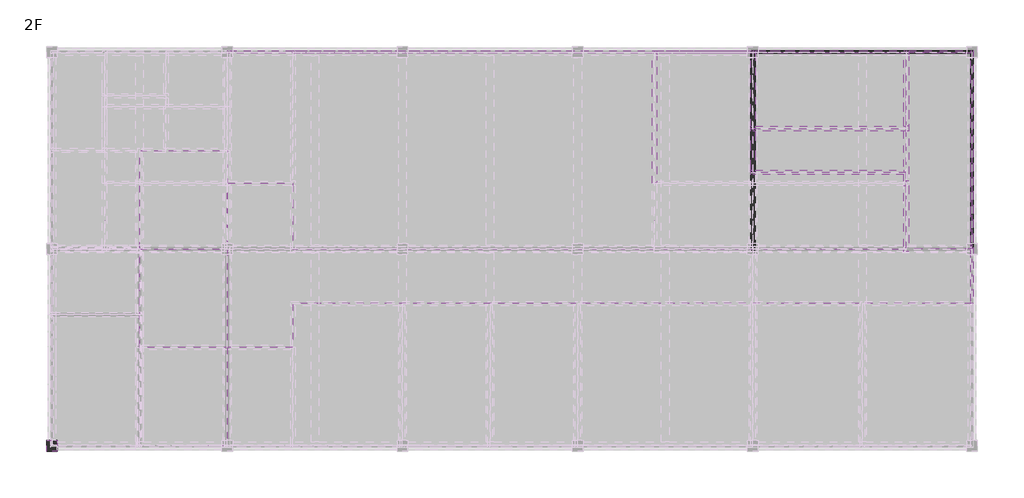
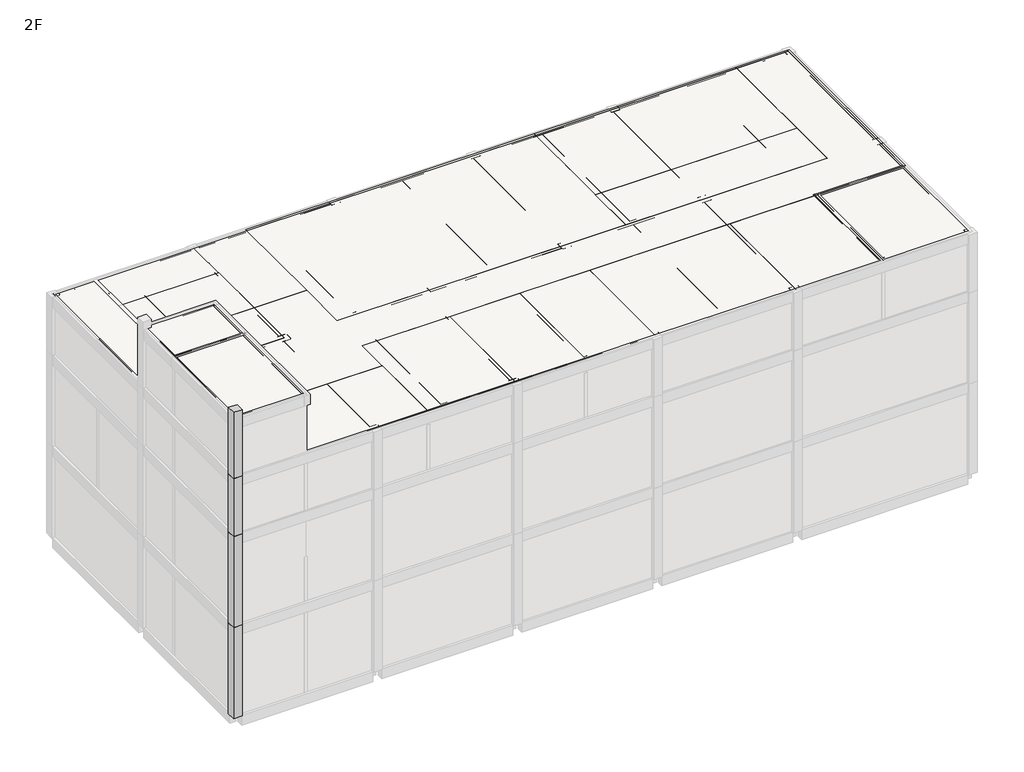
# One storey, part 3 of 7: 58 slabs, 19 walls, 4 columns.
"""IFC4 building model written with IfcOpenShell, lengths in millimetres."""

import ifcopenshell
import ifcopenshell.guid

model = None  # the IFC model being written
_history = None  # IfcOwnerHistory: only IFC2X3 demands one
_inside = {}  # id of a spatial element -> (the spatial element, [elements in it])
_under = {}  # id of a project, library or spatial element -> (it, [spatial elements below it])
_declared = {}  # id of a project -> (the project, [libraries it declares])
_typed = {}  # id of a type object -> (the type object, [elements of that type])
_made_of = {}  # id of a material, layer set ... -> (it, [elements and type objects made of it])


def new_model(schema):
    """Start an empty IFC model of exactly this schema.

    Asked for "IFC4X3", IfcOpenShell would pick the latest addendum, in which some entities
    have other attributes; the version numbers below select the first issue.
    IFC2X3 requires an IfcOwnerHistory on every rooted entity: one is made here for all.
    """
    global model, _history
    if schema == "IFC4X3":
        model = ifcopenshell.file(schema_version=(4, 3, 0, 0))
    else:
        model = ifcopenshell.file(schema=schema)
    _inside.clear()
    _under.clear()
    _declared.clear()
    _typed.clear()
    _made_of.clear()
    _history = None
    if model.schema == "IFC2X3":
        org = make("IfcOrganization", Name="unknown")
        user = make(
            "IfcPersonAndOrganization",
            ThePerson=make("IfcPerson", FamilyName="unknown"),
            TheOrganization=org,
        )
        app = make(
            "IfcApplication",
            ApplicationDeveloper=org,
            Version="unknown",
            ApplicationFullName="unknown",
            ApplicationIdentifier="unknown",
        )
        _history = make(
            "IfcOwnerHistory",
            OwningUser=user,
            OwningApplication=app,
            ChangeAction="ADDED",
            CreationDate=0,
        )
    return model


def make(cls, **values):
    """One entity of the class cls with the attributes given. An attribute that is None is left unset."""
    return model.create_entity(
        cls, **{name: value for name, value in values.items() if value is not None}
    )


def rooted(cls, **values):
    """An entity with a GlobalId (a new one), such as an element, a storey or a relation."""
    return make(cls, GlobalId=ifcopenshell.guid.new(), OwnerHistory=_history, **values)


def si_unit(unit_type, name, prefix=None):
    """IfcSIUnit, for example si_unit("LENGTHUNIT", "METRE", prefix="MILLI")."""
    return make("IfcSIUnit", UnitType=unit_type, Prefix=prefix, Name=name)


def assignment(units):
    """IfcUnitAssignment: the units of a project."""
    return None if units is None else make("IfcUnitAssignment", Units=units)


def point(xyz):
    """IfcCartesianPoint."""
    return None if xyz is None else make("IfcCartesianPoint", Coordinates=xyz)


def direction(xyz):
    """IfcDirection."""
    return None if xyz is None else make("IfcDirection", DirectionRatios=xyz)


def frame(location, z_axis=None, x_axis=None):
    """IfcAxis2Placement3D, a coordinate frame: its origin and axes. An axis left out is left unset."""
    return make(
        "IfcAxis2Placement3D",
        Location=point(location),
        Axis=direction(z_axis),
        RefDirection=direction(x_axis),
    )


def origin():
    """The frame at (0, 0, 0) with its axes left unset."""
    return frame((0.0, 0.0, 0.0))


def place(relative_to, where):
    """IfcLocalPlacement: puts the frame where relative to a parent placement (None: the world)."""
    return make(
        "IfcLocalPlacement", PlacementRelTo=relative_to, RelativePlacement=where
    )


def context(
    kind, dimensions, precision=None, world=None, true_north=None, identifier=None
):
    """IfcGeometricRepresentationContext, for example the 3D "Model" context."""
    return make(
        "IfcGeometricRepresentationContext",
        ContextIdentifier=identifier,
        ContextType=kind,
        CoordinateSpaceDimension=dimensions,
        Precision=precision,
        WorldCoordinateSystem=world,
        TrueNorth=true_north,
    )


def project(units=None, contexts=None):
    """IfcProject with its units and contexts."""
    return rooted(
        "IfcProject",
        Name="project",
        RepresentationContexts=contexts,
        UnitsInContext=assignment(units),
    )


def spatial(cls, under=None, at=None, **own):
    """A site, building, storey or space (cls), placed at a placement, below another one or the project."""
    s = rooted(cls, ObjectPlacement=at, **own)
    if under is not None:
        _under.setdefault(under.id(), (under, []))[1].append(s)
    return s


def polyline(points):
    """IfcPolyline through the points."""
    return make("IfcPolyline", Points=[point(p) for p in points])


def outline(outer, holes=None, kind="AREA"):
    """IfcArbitraryClosedProfileDef: a profile drawn as a closed curve; with holes, ...WithVoids."""
    if holes is None:
        return make("IfcArbitraryClosedProfileDef", ProfileType=kind, OuterCurve=outer)
    return make(
        "IfcArbitraryProfileDefWithVoids",
        ProfileType=kind,
        OuterCurve=outer,
        InnerCurves=holes,
    )


def extrude(swept, where, along, depth):
    """IfcExtrudedAreaSolid: the profile swept, set in the frame where, extruded along a direction by depth."""
    return make(
        "IfcExtrudedAreaSolid",
        SweptArea=swept,
        Position=where,
        ExtrudedDirection=direction(along),
        Depth=depth,
    )


def faces_of(points, faces, orient=None, outer=None):
    """IfcFace entities. A face is a list of loops; a loop is a list of indices into points, from 0.

    orient and outer hold one flag for each loop. By default every Orientation is true, the
    first loop of a face is its IfcFaceOuterBound and the others are IfcFaceBound.
    """
    made = []
    for i, loops in enumerate(faces):
        bounds = []
        for j, loop in enumerate(loops):
            is_outer = j == 0 if outer is None else outer[i][j]
            bounds.append(
                make(
                    "IfcFaceOuterBound" if is_outer else "IfcFaceBound",
                    Bound=make("IfcPolyLoop", Polygon=[points[k] for k in loop]),
                    Orientation=True if orient is None else orient[i][j],
                )
            )
        made.append(make("IfcFace", Bounds=bounds))
    return made


def faceted_brep(points, faces, orient=None, outer=None, voids=None):
    """IfcFacetedBrep: a solid bounded by flat faces; with voids (closed shells), ...WithVoids."""
    shared = [point(p) for p in points]
    hull = make("IfcClosedShell", CfsFaces=faces_of(shared, faces, orient, outer))
    if voids is None:
        return make("IfcFacetedBrep", Outer=hull)
    return make(
        "IfcFacetedBrepWithVoids",
        Outer=hull,
        Voids=[
            make(cls, CfsFaces=faces_of(shared, fs, o, b)) for cls, fs, o, b in voids
        ],
    )


def shape(context_of_items, identifier, shape_type, items):
    """IfcShapeRepresentation: the items that make up one representation, for example the "Body"."""
    return make(
        "IfcShapeRepresentation",
        ContextOfItems=context_of_items,
        RepresentationIdentifier=identifier,
        RepresentationType=shape_type,
        Items=items,
    )


def made_of(thing, what):
    """Note that an element or type object is made of a material, layer set ...; save() writes the relation."""
    if what is not None:
        _made_of.setdefault(what.id(), (what, []))[1].append(thing)
    return thing


def element(
    cls,
    number,
    at=None,
    inside=None,
    cuts=None,
    type_object=None,
    material=None,
    context=None,
    identifier="Body",
    shape_type=None,
    held_by="IfcProductDefinitionShape",
    body=None,
    shapes=None,
    **own,
):
    """One element of the class cls, such as IfcWall. Its Tag is "e" and its number.

    at: its placement. inside: the storey or other place that contains it. cuts: it is an
    opening in that element (IfcRelVoidsElement). A single representation is given by context,
    identifier, shape_type and body (its items); several are given by shapes. held_by: the class
    of the entity that holds the representations. save() writes the other relations.
    """
    e = rooted(cls, Tag="e%d" % number, ObjectPlacement=at, **own)
    if body is not None:
        shapes = [shape(context, identifier, shape_type, body)]
    if shapes is not None:
        e.Representation = make(held_by, Representations=shapes)
    if inside is not None:
        _inside.setdefault(inside.id(), (inside, []))[1].append(e)
    if cuts is not None:
        rooted(
            "IfcRelVoidsElement", RelatingBuildingElement=cuts, RelatedOpeningElement=e
        )
    if type_object is not None:
        _typed.setdefault(type_object.id(), (type_object, []))[1].append(e)
    return made_of(e, material)


def aggregate(whole, parts):
    """IfcRelAggregates: a whole, such as a stair, and the parts it consists of."""
    return rooted("IfcRelAggregates", RelatingObject=whole, RelatedObjects=parts)


def save(model, path):
    """Write the relations noted so far, then the file.

    IfcRelAggregates (storeys below a building ...), IfcRelContainedInSpatialStructure (elements
    in a storey), IfcRelDefinesByType, IfcRelAssociatesMaterial and IfcRelDeclares: one each for
    every whole, place, type object, material and project.
    """
    for whole, parts in _under.values():
        aggregate(whole, parts)
    for where, things in _inside.values():
        rooted(
            "IfcRelContainedInSpatialStructure",
            RelatedElements=things,
            RelatingStructure=where,
        )
    for kind, things in _typed.values():
        rooted("IfcRelDefinesByType", RelatedObjects=things, RelatingType=kind)
    for what, things in _made_of.values():
        rooted("IfcRelAssociatesMaterial", RelatedObjects=things, RelatingMaterial=what)
    for by, libraries in _declared.values():
        rooted("IfcRelDeclares", RelatingContext=by, RelatedDefinitions=libraries)
    model.write(path)


model = new_model("IFC4")

# Units and contexts
model_context = context("Model", 3, world=origin())
ifc_project = project(units=[si_unit("LENGTHUNIT", "METRE", prefix="MILLI")], contexts=[model_context])

# Site, building, storey
site = spatial("IfcSite", under=ifc_project)
building = spatial("IfcBuilding", under=site)
storey = spatial("IfcBuildingStorey", under=building, Name="2F", Elevation=3500.0)

# Columns
placement = place(None, origin())
element("IfcColumn", 1, ObjectType="Concrete-Rectangular-Column : CL111_500x500", at=placement, inside=storey, context=model_context, shape_type="SweptSolid", body=[
    extrude(outline(polyline([(45709.6521483, 164173.8614395), (45709.6521483, 163673.8614395), (45209.6521483, 163673.8614395), (45209.6521483, 164173.8614395), (45709.6521483, 164173.8614395)])), frame((0.0, 0.0, 18000.0), z_axis=(0.0, 0.0, 1.0), x_axis=(1.0, 0.0, 0.0)), (0.0, 0.0, 1.0), 4000.0),
])
element("IfcColumn", 2, ObjectType="Concrete-Rectangular-Column : CL111_500x500", at=placement, inside=storey, context=model_context, shape_type="Brep", body=[
    faceted_brep([(45709.6521483, 164173.8614395, 3500.0), (45709.6521483, 163673.8614395, 3500.0), (45209.6521483, 163673.8614395, 3500.0), (45209.6521483, 164173.8614395, 3500.0), (45709.6521483, 164173.8614395, 9000.0), (45709.6521483, 164098.8614395, 9000.0), (45709.6521483, 163748.8614395, 9000.0), (45709.6521483, 163673.8614395, 9000.0), (45209.6521483, 163673.8614395, 9000.0), (45209.6521483, 164173.8614395, 9000.0), (45284.6521483, 164173.8614395, 9000.0), (45634.6521483, 164173.8614395, 9000.0)], [[[0, 1, 2, 3]], [[4, 5, 6, 7, 1, 0]], [[7, 8, 2, 1]], [[8, 9, 3, 2]], [[9, 10, 11, 4, 0, 3]], [[4, 11, 10, 9, 8, 7, 6, 5]]]),
])
element("IfcColumn", 3, ObjectType="Concrete-Rectangular-Column : CL111_500x500", at=placement, inside=storey, context=model_context, shape_type="Brep", body=[
    faceted_brep([(45709.6521483, 164173.8614395, 9000.0), (45709.6521483, 163673.8614395, 9000.0), (45209.6521483, 163673.8614395, 9000.0), (45209.6521483, 164173.8614395, 9000.0), (45709.6521483, 164173.8614395, 14500.0), (45709.6521483, 164098.8614395, 14500.0), (45709.6521483, 163748.8614395, 14500.0), (45709.6521483, 163673.8614395, 14500.0), (45209.6521483, 163673.8614395, 14500.0), (45209.6521483, 164173.8614395, 14500.0), (45284.6521483, 164173.8614395, 14500.0), (45634.6521483, 164173.8614395, 14500.0)], [[[0, 1, 2, 3]], [[4, 5, 6, 7, 1, 0]], [[7, 8, 2, 1]], [[8, 9, 3, 2]], [[9, 10, 11, 4, 0, 3]], [[4, 11, 10, 9, 8, 7, 6, 5]]]),
])
element("IfcColumn", 4, ObjectType="Concrete-Rectangular-Column : CL111_500x500", at=placement, inside=storey, context=model_context, shape_type="Brep", body=[
    faceted_brep([(45709.6521483, 164173.8614395, 14500.0), (45709.6521483, 163673.8614395, 14500.0), (45209.6521483, 163673.8614395, 14500.0), (45209.6521483, 164173.8614395, 14500.0), (45709.6521483, 164173.8614395, 18000.0), (45709.6521483, 164098.8614395, 18000.0), (45709.6521483, 163748.8614395, 18000.0), (45709.6521483, 163673.8614395, 18000.0), (45209.6521483, 163673.8614395, 18000.0), (45209.6521483, 164173.8614395, 18000.0), (45284.6521483, 164173.8614395, 18000.0), (45634.6521483, 164173.8614395, 18000.0)], [[[0, 1, 2, 3]], [[4, 5, 6, 7, 1, 0]], [[7, 8, 2, 1]], [[8, 9, 3, 2]], [[9, 10, 11, 4, 0, 3]], [[4, 11, 10, 9, 8, 7, 6, 5]]]),
])

# Slabs
element("IfcSlab", 5, ObjectType="CFS11_Slab RC_T150", at=placement, inside=storey, context=model_context, shape_type="SweptSolid", body=[
    extrude(outline(polyline([(77459.6521483, 181923.8614395), (77459.6521483, 172923.8614395), (45459.6521483, 172923.8614395), (45459.6521483, 181923.8614395), (77459.6521483, 181923.8614395)])), frame((0.0, 0.0, 3350.0), z_axis=(0.0, 0.0, 1.0), x_axis=(1.0, 0.0, 0.0)), (0.0, 0.0, 1.0), 150.0),
])
element("IfcSlab", 6, ObjectType="CFS11_Slab RC_T150", at=placement, inside=storey, context=model_context, shape_type="SweptSolid", body=[
    extrude(outline(polyline([(53459.6521483, 163923.8614395), (53459.6521483, 172923.8614395), (87459.6521483, 172923.8614395), (87459.6521483, 163923.8614395), (53459.6521483, 163923.8614395)])), frame((0.0, 0.0, 3350.0), z_axis=(0.0, 0.0, 1.0), x_axis=(1.0, 0.0, 0.0)), (0.0, 0.0, 1.0), 150.0),
])
element("IfcSlab", 7, ObjectType="CFS11_Slab RC_T150", at=placement, inside=storey, context=model_context, shape_type="SweptSolid", body=[
    extrude(outline(polyline([(77459.6521483, 181923.8614395), (87459.6521483, 181923.8614395), (87459.6521483, 172923.8614395), (77459.6521483, 172923.8614395), (77459.6521483, 181923.8614395)])), frame((0.0, 0.0, 3350.0), z_axis=(0.0, 0.0, 1.0), x_axis=(1.0, 0.0, 0.0)), (0.0, 0.0, 1.0), 150.0),
])
element("IfcSlab", 8, ObjectType="CFS11_Slab RC_T150", at=placement, inside=storey, context=model_context, shape_type="SweptSolid", body=[
    extrude(outline(polyline([(53459.6521483, 172923.8614395), (53459.6521483, 163923.8614395), (49459.6521483, 163923.8614395), (49459.6521483, 172923.8614395), (53459.6521483, 172923.8614395)])), frame((0.0, 0.0, 3350.0), z_axis=(0.0, 0.0, 1.0), x_axis=(1.0, 0.0, 0.0)), (0.0, 0.0, 1.0), 150.0),
])
element("IfcSlab", 9, ObjectType="CFS11_Slab RC_T150", at=placement, inside=storey, context=model_context, shape_type="SweptSolid", body=[
    extrude(outline(polyline([(49459.6521483, 172923.8614395), (49459.6521483, 169923.8614395), (45459.6521483, 169923.8614395), (45459.6521483, 172923.8614395), (49459.6521483, 172923.8614395)])), frame((0.0, 0.0, 3350.0), z_axis=(0.0, 0.0, 1.0), x_axis=(1.0, 0.0, 0.0)), (0.0, 0.0, 1.0), 150.0),
])
element("IfcSlab", 10, ObjectType="CFS11_Slab RC_T150", at=placement, inside=storey, context=model_context, shape_type="SweptSolid", body=[
    extrude(outline(polyline([(49459.6521483, 163923.8614395), (45459.6521483, 163923.8614395), (45459.6521483, 169923.8614395), (49459.6521483, 169923.8614395), (49459.6521483, 163923.8614395)])), frame((0.0, 0.0, 3350.0), z_axis=(0.0, 0.0, 1.0), x_axis=(1.0, 0.0, 0.0)), (0.0, 0.0, 1.0), 150.0),
])
element("IfcSlab", 11, ObjectType="CFS11_Slab RC_T150", at=placement, inside=storey, context=model_context, shape_type="SweptSolid", body=[
    extrude(outline(polyline([(53459.6521483, 181923.8614395), (77459.6521483, 181923.8614395), (77459.6521483, 172923.8614395), (53459.6521483, 172923.8614395), (53459.6521483, 181923.8614395)])), frame((0.0, 0.0, 8850.0), z_axis=(0.0, 0.0, 1.0), x_axis=(1.0, 0.0, 0.0)), (0.0, 0.0, 1.0), 150.0),
])
element("IfcSlab", 12, ObjectType="CFS11_Slab RC_T150", at=placement, inside=storey, context=model_context, shape_type="SweptSolid", body=[
    extrude(outline(polyline([(77459.6521483, 172923.8614395), (77459.6521483, 163923.8614395), (53459.6521483, 163923.8614395), (53459.6521483, 172923.8614395), (77459.6521483, 172923.8614395)])), frame((0.0, 0.0, 8850.0), z_axis=(0.0, 0.0, 1.0), x_axis=(1.0, 0.0, 0.0)), (0.0, 0.0, 1.0), 150.0),
])
element("IfcSlab", 13, ObjectType="CFS11_Slab RC_T150", at=placement, inside=storey, context=model_context, shape_type="SweptSolid", body=[
    extrude(outline(polyline([(77459.6521483, 181923.8614395), (84459.6521483, 181923.8614395), (84459.6521483, 178423.8614395), (77459.6521483, 178423.8614395), (77459.6521483, 181923.8614395)])), frame((0.0, 0.0, 8850.0), z_axis=(0.0, 0.0, 1.0), x_axis=(1.0, 0.0, 0.0)), (0.0, 0.0, 1.0), 150.0),
])
element("IfcSlab", 14, ObjectType="CFS11_Slab RC_T150", at=placement, inside=storey, context=model_context, shape_type="SweptSolid", body=[
    extrude(outline(polyline([(77459.6521483, 163923.8614395), (77459.6521483, 172923.8614395), (87459.6521483, 172923.8614395), (87459.6521483, 163923.8614395), (77459.6521483, 163923.8614395)])), frame((0.0, 0.0, 8850.0), z_axis=(0.0, 0.0, 1.0), x_axis=(1.0, 0.0, 0.0)), (0.0, 0.0, 1.0), 150.0),
])
element("IfcSlab", 15, ObjectType="CFS11_Slab RC_T150", at=placement, inside=storey, context=model_context, shape_type="SweptSolid", body=[
    extrude(outline(polyline([(77459.6521483, 176423.8614395), (84459.6521483, 176423.8614395), (84459.6521483, 172923.8614395), (77459.6521483, 172923.8614395), (77459.6521483, 176423.8614395)])), frame((0.0, 0.0, 8850.0), z_axis=(0.0, 0.0, 1.0), x_axis=(1.0, 0.0, 0.0)), (0.0, 0.0, 1.0), 150.0),
])
element("IfcSlab", 16, ObjectType="CFS11_Slab RC_T150", at=placement, inside=storey, context=model_context, shape_type="SweptSolid", body=[
    extrude(outline(polyline([(45459.6521483, 181923.8614395), (47859.6521483, 181923.8614395), (47859.6521483, 177423.8614395), (45459.6521483, 177423.8614395), (45459.6521483, 181923.8614395)])), frame((0.0, 0.0, 8850.0), z_axis=(0.0, 0.0, 1.0), x_axis=(1.0, 0.0, 0.0)), (0.0, 0.0, 1.0), 150.0),
])
element("IfcSlab", 17, ObjectType="CFS11_Slab RC_T150", at=placement, inside=storey, context=model_context, shape_type="SweptSolid", body=[
    extrude(outline(polyline([(45459.6521483, 172923.8614395), (45459.6521483, 177423.8614395), (49459.6521483, 177423.8614395), (49459.6521483, 172923.8614395), (45459.6521483, 172923.8614395)])), frame((0.0, 0.0, 8850.0), z_axis=(0.0, 0.0, 1.0), x_axis=(1.0, 0.0, 0.0)), (0.0, 0.0, 1.0), 150.0),
])
element("IfcSlab", 18, ObjectType="CFS11_Slab RC_T150", at=placement, inside=storey, context=model_context, shape_type="SweptSolid", body=[
    extrude(outline(polyline([(53459.6521483, 177423.8614395), (50659.6521483, 177423.8614395), (50659.6521483, 181923.8614395), (53459.6521483, 181923.8614395), (53459.6521483, 177423.8614395)])), frame((0.0, 0.0, 8850.0), z_axis=(0.0, 0.0, 1.0), x_axis=(1.0, 0.0, 0.0)), (0.0, 0.0, 1.0), 150.0),
])
element("IfcSlab", 19, ObjectType="CFS11_Slab RC_T150", at=placement, inside=storey, context=model_context, shape_type="SweptSolid", body=[
    extrude(outline(polyline([(47859.6521483, 181923.8614395), (50659.6521483, 181923.8614395), (50659.6521483, 179923.8614395), (47859.6521483, 179923.8614395), (47859.6521483, 181923.8614395)])), frame((0.0, 0.0, 8850.0), z_axis=(0.0, 0.0, 1.0), x_axis=(1.0, 0.0, 0.0)), (0.0, 0.0, 1.0), 150.0),
])
element("IfcSlab", 20, ObjectType="CFS11_Slab RC_T150", at=placement, inside=storey, context=model_context, shape_type="SweptSolid", body=[
    extrude(outline(polyline([(47859.6521483, 179923.8614395), (50659.6521483, 179923.8614395), (50659.6521483, 177423.8614395), (47859.6521483, 177423.8614395), (47859.6521483, 179923.8614395)])), frame((0.0, 0.0, 8850.0), z_axis=(0.0, 0.0, 1.0), x_axis=(1.0, 0.0, 0.0)), (0.0, 0.0, 1.0), 150.0),
])
element("IfcSlab", 21, ObjectType="CFS11_Slab RC_T150", at=placement, inside=storey, context=model_context, shape_type="SweptSolid", body=[
    extrude(outline(polyline([(49459.6521483, 172923.8614395), (49459.6521483, 169923.8614395), (45459.6521483, 169923.8614395), (45459.6521483, 172923.8614395), (49459.6521483, 172923.8614395)])), frame((0.0, 0.0, 8850.0), z_axis=(0.0, 0.0, 1.0), x_axis=(1.0, 0.0, 0.0)), (0.0, 0.0, 1.0), 150.0),
])
element("IfcSlab", 22, ObjectType="CFS11_Slab RC_T150", at=placement, inside=storey, context=model_context, shape_type="SweptSolid", body=[
    extrude(outline(polyline([(49459.6521483, 169923.8614395), (49459.6521483, 163923.8614395), (45459.6521483, 163923.8614395), (45459.6521483, 169923.8614395), (49459.6521483, 169923.8614395)])), frame((0.0, 0.0, 8850.0), z_axis=(0.0, 0.0, 1.0), x_axis=(1.0, 0.0, 0.0)), (0.0, 0.0, 1.0), 150.0),
])
element("IfcSlab", 23, ObjectType="CFS11_Slab RC_T150", at=placement, inside=storey, context=model_context, shape_type="SweptSolid", body=[
    extrude(outline(polyline([(77459.6521483, 178423.8614395), (84459.6521483, 178423.8614395), (84459.6521483, 181923.8614395), (87459.6521483, 181923.8614395), (87459.6521483, 172923.8614395), (84459.6521483, 172923.8614395), (84459.6521483, 176423.8614395), (77459.6521483, 176423.8614395), (77459.6521483, 178423.8614395)])), frame((0.0, 0.0, 8850.0), z_axis=(0.0, 0.0, 1.0), x_axis=(1.0, 0.0, 0.0)), (0.0, 0.0, 1.0), 150.0),
])
element("IfcSlab", 24, ObjectType="CFS11_Slab RC_T150", at=placement, inside=storey, context=model_context, shape_type="SweptSolid", body=[
    extrude(outline(polyline([(49459.6521483, 177423.8614395), (53459.6521483, 177423.8614395), (53459.6521483, 163923.8614395), (49459.6521483, 163923.8614395), (49459.6521483, 177423.8614395)])), frame((0.0, 0.0, 8850.0), z_axis=(0.0, 0.0, 1.0), x_axis=(1.0, 0.0, 0.0)), (0.0, 0.0, 1.0), 150.0),
])
element("IfcSlab", 25, ObjectType="CFS11_Slab RC_T150", at=placement, inside=storey, context=model_context, shape_type="SweptSolid", body=[
    extrude(outline(polyline([(61459.6521483, 163923.8614395), (61459.6521483, 170423.8614395), (65459.6521483, 170423.8614395), (65459.6521483, 163923.8614395), (61459.6521483, 163923.8614395)])), frame((0.0, 0.0, 14350.0), z_axis=(0.0, 0.0, 1.0), x_axis=(1.0, 0.0, 0.0)), (0.0, 0.0, 1.0), 150.0),
])
element("IfcSlab", 26, ObjectType="CFS11_Slab RC_T150", at=placement, inside=storey, context=model_context, shape_type="SweptSolid", body=[
    extrude(outline(polyline([(65459.6521483, 170423.8614395), (69459.6521483, 170423.8614395), (69459.6521483, 163923.8614395), (65459.6521483, 163923.8614395), (65459.6521483, 170423.8614395)])), frame((0.0, 0.0, 14350.0), z_axis=(0.0, 0.0, 1.0), x_axis=(1.0, 0.0, 0.0)), (0.0, 0.0, 1.0), 150.0),
])
element("IfcSlab", 27, ObjectType="CFS11_Slab RC_T150", at=placement, inside=storey, context=model_context, shape_type="SweptSolid", body=[
    extrude(outline(polyline([(84459.6521483, 181923.8614395), (84459.6521483, 175923.8614395), (72959.6521483, 175923.8614395), (72959.6521483, 181923.8614395), (84459.6521483, 181923.8614395)])), frame((0.0, 0.0, 14350.0), z_axis=(0.0, 0.0, 1.0), x_axis=(1.0, 0.0, 0.0)), (0.0, 0.0, 1.0), 150.0),
])
element("IfcSlab", 28, ObjectType="CFS11_Slab RC_T150", at=placement, inside=storey, context=model_context, shape_type="SweptSolid", body=[
    extrude(outline(polyline([(69459.6521483, 170423.8614395), (77459.6521483, 170423.8614395), (77459.6521483, 163923.8614395), (69459.6521483, 163923.8614395), (69459.6521483, 170423.8614395)])), frame((0.0, 0.0, 14350.0), z_axis=(0.0, 0.0, 1.0), x_axis=(1.0, 0.0, 0.0)), (0.0, 0.0, 1.0), 150.0),
])
element("IfcSlab", 29, ObjectType="CFS11_Slab RC_T150", at=placement, inside=storey, context=model_context, shape_type="SweptSolid", body=[
    extrude(outline(polyline([(56459.6521483, 181923.8614395), (72959.6521483, 181923.8614395), (72959.6521483, 172923.8614395), (56459.6521483, 172923.8614395), (56459.6521483, 181923.8614395)])), frame((0.0, 0.0, 14350.0), z_axis=(0.0, 0.0, 1.0), x_axis=(1.0, 0.0, 0.0)), (0.0, 0.0, 1.0), 150.0),
])
element("IfcSlab", 30, ObjectType="CFS11_Slab RC_T150", at=placement, inside=storey, context=model_context, shape_type="SweptSolid", body=[
    extrude(outline(polyline([(77459.6521483, 170423.8614395), (82459.6521483, 170423.8614395), (82459.6521483, 163923.8614395), (77459.6521483, 163923.8614395), (77459.6521483, 170423.8614395)])), frame((0.0, 0.0, 14350.0), z_axis=(0.0, 0.0, 1.0), x_axis=(1.0, 0.0, 0.0)), (0.0, 0.0, 1.0), 150.0),
])
element("IfcSlab", 31, ObjectType="CFS11_Slab RC_T150", at=placement, inside=storey, context=model_context, shape_type="SweptSolid", body=[
    extrude(outline(polyline([(82459.6521483, 170423.8614395), (87459.6521483, 170423.8614395), (87459.6521483, 163923.8614395), (82459.6521483, 163923.8614395), (82459.6521483, 170423.8614395)])), frame((0.0, 0.0, 14350.0), z_axis=(0.0, 0.0, 1.0), x_axis=(1.0, 0.0, 0.0)), (0.0, 0.0, 1.0), 150.0),
])
element("IfcSlab", 32, ObjectType="CFS11_Slab RC_T150", at=placement, inside=storey, context=model_context, shape_type="SweptSolid", body=[
    extrude(outline(polyline([(84459.6521483, 175923.8614395), (84459.6521483, 172923.8614395), (72959.6521483, 172923.8614395), (72959.6521483, 175923.8614395), (84459.6521483, 175923.8614395)])), frame((0.0, 0.0, 14350.0), z_axis=(0.0, 0.0, 1.0), x_axis=(1.0, 0.0, 0.0)), (0.0, 0.0, 1.0), 150.0),
])
element("IfcSlab", 33, ObjectType="CFS11_Slab RC_T150", at=placement, inside=storey, context=model_context, shape_type="SweptSolid", body=[
    extrude(outline(polyline([(61459.6521483, 163923.8614395), (56459.6521483, 163923.8614395), (56459.6521483, 170423.8614395), (61459.6521483, 170423.8614395), (61459.6521483, 163923.8614395)])), frame((0.0, 0.0, 14350.0), z_axis=(0.0, 0.0, 1.0), x_axis=(1.0, 0.0, 0.0)), (0.0, 0.0, 1.0), 150.0),
])
element("IfcSlab", 34, ObjectType="CFS11_Slab RC_T150", at=placement, inside=storey, context=model_context, shape_type="SweptSolid", body=[
    extrude(outline(polyline([(56459.6521483, 163923.8614395), (49459.6521483, 163923.8614395), (49459.6521483, 168423.8614395), (56459.6521483, 168423.8614395), (56459.6521483, 163923.8614395)])), frame((0.0, 0.0, 14350.0), z_axis=(0.0, 0.0, 1.0), x_axis=(1.0, 0.0, 0.0)), (0.0, 0.0, 1.0), 150.0),
])
element("IfcSlab", 35, ObjectType="CFS11_Slab RC_T150", at=placement, inside=storey, context=model_context, shape_type="SweptSolid", body=[
    extrude(outline(polyline([(53459.6521483, 179423.8614395), (53459.6521483, 175923.8614395), (47859.6521483, 175923.8614395), (47859.6521483, 179423.8614395), (53459.6521483, 179423.8614395)])), frame((0.0, 0.0, 14350.0), z_axis=(0.0, 0.0, 1.0), x_axis=(1.0, 0.0, 0.0)), (0.0, 0.0, 1.0), 150.0),
])
element("IfcSlab", 36, ObjectType="CFS11_Slab RC_T150", at=placement, inside=storey, context=model_context, shape_type="SweptSolid", body=[
    extrude(outline(polyline([(47859.6521483, 179423.8614395), (47859.6521483, 181923.8614395), (53459.6521483, 181923.8614395), (53459.6521483, 179423.8614395), (47859.6521483, 179423.8614395)])), frame((0.0, 0.0, 14350.0), z_axis=(0.0, 0.0, 1.0), x_axis=(1.0, 0.0, 0.0)), (0.0, 0.0, 1.0), 150.0),
])
element("IfcSlab", 37, ObjectType="CFS11_Slab RC_T150", at=placement, inside=storey, context=model_context, shape_type="SweptSolid", body=[
    extrude(outline(polyline([(56459.6521483, 175923.8614395), (53459.6521483, 175923.8614395), (53459.6521483, 181923.8614395), (56459.6521483, 181923.8614395), (56459.6521483, 175923.8614395)])), frame((0.0, 0.0, 14350.0), z_axis=(0.0, 0.0, 1.0), x_axis=(1.0, 0.0, 0.0)), (0.0, 0.0, 1.0), 150.0),
])
element("IfcSlab", 38, ObjectType="CFS11_Slab RC_T150", at=placement, inside=storey, context=model_context, shape_type="SweptSolid", body=[
    extrude(outline(polyline([(53459.6521483, 175923.8614395), (53459.6521483, 172923.8614395), (47859.6521483, 172923.8614395), (47859.6521483, 175923.8614395), (53459.6521483, 175923.8614395)])), frame((0.0, 0.0, 14350.0), z_axis=(0.0, 0.0, 1.0), x_axis=(1.0, 0.0, 0.0)), (0.0, 0.0, 1.0), 150.0),
])
element("IfcSlab", 39, ObjectType="CFS11_Slab RC_T150", at=placement, inside=storey, context=model_context, shape_type="SweptSolid", body=[
    extrude(outline(polyline([(45459.6521483, 181923.8614395), (47859.6521483, 181923.8614395), (47859.6521483, 172923.8614395), (45459.6521483, 172923.8614395), (45459.6521483, 181923.8614395)])), frame((0.0, 0.0, 14350.0), z_axis=(0.0, 0.0, 1.0), x_axis=(1.0, 0.0, 0.0)), (0.0, 0.0, 1.0), 150.0),
])
element("IfcSlab", 40, ObjectType="CFS11_Slab RC_T150", at=placement, inside=storey, context=model_context, shape_type="SweptSolid", body=[
    extrude(outline(polyline([(49459.6521483, 172923.8614395), (49459.6521483, 169923.8614395), (45459.6521483, 169923.8614395), (45459.6521483, 172923.8614395), (49459.6521483, 172923.8614395)])), frame((0.0, 0.0, 14350.0), z_axis=(0.0, 0.0, 1.0), x_axis=(1.0, 0.0, 0.0)), (0.0, 0.0, 1.0), 150.0),
])
element("IfcSlab", 41, ObjectType="CFS11_Slab RC_T150", at=placement, inside=storey, context=model_context, shape_type="SweptSolid", body=[
    extrude(outline(polyline([(49459.6521483, 163923.8614395), (45459.6521483, 163923.8614395), (45459.6521483, 169923.8614395), (49459.6521483, 169923.8614395), (49459.6521483, 163923.8614395)])), frame((0.0, 0.0, 14350.0), z_axis=(0.0, 0.0, 1.0), x_axis=(1.0, 0.0, 0.0)), (0.0, 0.0, 1.0), 150.0),
])
element("IfcSlab", 42, ObjectType="CFS11_Slab RC_T150", at=placement, inside=storey, context=model_context, shape_type="SweptSolid", body=[
    extrude(outline(polyline([(87459.6521483, 181923.8614395), (87459.6521483, 170423.8614395), (56459.6521483, 170423.8614395), (56459.6521483, 168423.8614395), (49459.6521483, 168423.8614395), (49459.6521483, 172923.8614395), (53459.6521483, 172923.8614395), (53459.6521483, 175923.8614395), (56459.6521483, 175923.8614395), (56459.6521483, 172923.8614395), (84459.6521483, 172923.8614395), (84459.6521483, 181923.8614395), (87459.6521483, 181923.8614395)])), frame((0.0, 0.0, 14350.0), z_axis=(0.0, 0.0, 1.0), x_axis=(1.0, 0.0, 0.0)), (0.0, 0.0, 1.0), 150.0),
])
element("IfcSlab", 43, ObjectType="CFS11_Slab RC_T150", at=placement, inside=storey, context=model_context, shape_type="SweptSolid", body=[
    extrude(outline(polyline([(45459.6521483, 172923.8614395), (49459.6521483, 172923.8614395), (49459.6521483, 169923.8614395), (45459.6521483, 169923.8614395), (45459.6521483, 172923.8614395)])), frame((0.0, 0.0, 17850.0), z_axis=(0.0, 0.0, 1.0), x_axis=(1.0, 0.0, 0.0)), (0.0, 0.0, 1.0), 150.0),
])
element("IfcSlab", 44, ObjectType="CFS11_Slab RC_T150", at=placement, inside=storey, context=model_context, shape_type="SweptSolid", body=[
    extrude(outline(polyline([(49459.6521483, 169923.8614395), (49459.6521483, 163923.8614395), (45459.6521483, 163923.8614395), (45459.6521483, 169923.8614395), (49459.6521483, 169923.8614395)])), frame((0.0, 0.0, 17850.0), z_axis=(0.0, 0.0, 1.0), x_axis=(1.0, 0.0, 0.0)), (0.0, 0.0, 1.0), 150.0),
])
element("IfcSlab", 45, ObjectType="CFS11_Slab RC_T150", at=placement, inside=storey, context=model_context, shape_type="SweptSolid", body=[
    extrude(outline(polyline([(61459.6521483, 163923.8614395), (61459.6521483, 170423.8614395), (65459.6521483, 170423.8614395), (65459.6521483, 163923.8614395), (61459.6521483, 163923.8614395)])), frame((0.0, 0.0, 17850.0), z_axis=(0.0, 0.0, 1.0), x_axis=(1.0, 0.0, 0.0)), (0.0, 0.0, 1.0), 150.0),
])
element("IfcSlab", 46, ObjectType="CFS11_Slab RC_T150", at=placement, inside=storey, context=model_context, shape_type="SweptSolid", body=[
    extrude(outline(polyline([(65459.6521483, 170423.8614395), (69459.6521483, 170423.8614395), (69459.6521483, 163923.8614395), (65459.6521483, 163923.8614395), (65459.6521483, 170423.8614395)])), frame((0.0, 0.0, 17850.0), z_axis=(0.0, 0.0, 1.0), x_axis=(1.0, 0.0, 0.0)), (0.0, 0.0, 1.0), 150.0),
])
element("IfcSlab", 47, ObjectType="CFS11_Slab RC_T150", at=placement, inside=storey, context=model_context, shape_type="SweptSolid", body=[
    extrude(outline(polyline([(84459.6521483, 181923.8614395), (84459.6521483, 175923.8614395), (72959.6521483, 175923.8614395), (72959.6521483, 181923.8614395), (84459.6521483, 181923.8614395)])), frame((0.0, 0.0, 17850.0), z_axis=(0.0, 0.0, 1.0), x_axis=(1.0, 0.0, 0.0)), (0.0, 0.0, 1.0), 150.0),
])
element("IfcSlab", 48, ObjectType="CFS11_Slab RC_T150", at=placement, inside=storey, context=model_context, shape_type="SweptSolid", body=[
    extrude(outline(polyline([(69459.6521483, 170423.8614395), (77459.6521483, 170423.8614395), (77459.6521483, 163923.8614395), (69459.6521483, 163923.8614395), (69459.6521483, 170423.8614395)])), frame((0.0, 0.0, 17850.0), z_axis=(0.0, 0.0, 1.0), x_axis=(1.0, 0.0, 0.0)), (0.0, 0.0, 1.0), 150.0),
])
element("IfcSlab", 49, ObjectType="CFS11_Slab RC_T150", at=placement, inside=storey, context=model_context, shape_type="SweptSolid", body=[
    extrude(outline(polyline([(56459.6521483, 181923.8614395), (72959.6521483, 181923.8614395), (72959.6521483, 172923.8614395), (56459.6521483, 172923.8614395), (56459.6521483, 181923.8614395)])), frame((0.0, 0.0, 17850.0), z_axis=(0.0, 0.0, 1.0), x_axis=(1.0, 0.0, 0.0)), (0.0, 0.0, 1.0), 150.0),
])
element("IfcSlab", 50, ObjectType="CFS11_Slab RC_T150", at=placement, inside=storey, context=model_context, shape_type="SweptSolid", body=[
    extrude(outline(polyline([(77459.6521483, 170423.8614395), (82459.6521483, 170423.8614395), (82459.6521483, 163923.8614395), (77459.6521483, 163923.8614395), (77459.6521483, 170423.8614395)])), frame((0.0, 0.0, 17850.0), z_axis=(0.0, 0.0, 1.0), x_axis=(1.0, 0.0, 0.0)), (0.0, 0.0, 1.0), 150.0),
])
element("IfcSlab", 51, ObjectType="CFS11_Slab RC_T150", at=placement, inside=storey, context=model_context, shape_type="SweptSolid", body=[
    extrude(outline(polyline([(82459.6521483, 170423.8614395), (87459.6521483, 170423.8614395), (87459.6521483, 163923.8614395), (82459.6521483, 163923.8614395), (82459.6521483, 170423.8614395)])), frame((0.0, 0.0, 17850.0), z_axis=(0.0, 0.0, 1.0), x_axis=(1.0, 0.0, 0.0)), (0.0, 0.0, 1.0), 150.0),
])
element("IfcSlab", 52, ObjectType="CFS11_Slab RC_T150", at=placement, inside=storey, context=model_context, shape_type="SweptSolid", body=[
    extrude(outline(polyline([(84459.6521483, 175923.8614395), (84459.6521483, 172923.8614395), (72959.6521483, 172923.8614395), (72959.6521483, 175923.8614395), (84459.6521483, 175923.8614395)])), frame((0.0, 0.0, 17850.0), z_axis=(0.0, 0.0, 1.0), x_axis=(1.0, 0.0, 0.0)), (0.0, 0.0, 1.0), 150.0),
])
element("IfcSlab", 53, ObjectType="CFS11_Slab RC_T150", at=placement, inside=storey, context=model_context, shape_type="SweptSolid", body=[
    extrude(outline(polyline([(61459.6521483, 163923.8614395), (56459.6521483, 163923.8614395), (56459.6521483, 170423.8614395), (61459.6521483, 170423.8614395), (61459.6521483, 163923.8614395)])), frame((0.0, 0.0, 17850.0), z_axis=(0.0, 0.0, 1.0), x_axis=(1.0, 0.0, 0.0)), (0.0, 0.0, 1.0), 150.0),
])
element("IfcSlab", 54, ObjectType="CFS11_Slab RC_T150", at=placement, inside=storey, context=model_context, shape_type="SweptSolid", body=[
    extrude(outline(polyline([(56459.6521483, 163923.8614395), (49459.6521483, 163923.8614395), (49459.6521483, 168423.8614395), (56459.6521483, 168423.8614395), (56459.6521483, 163923.8614395)])), frame((0.0, 0.0, 17850.0), z_axis=(0.0, 0.0, 1.0), x_axis=(1.0, 0.0, 0.0)), (0.0, 0.0, 1.0), 150.0),
])
element("IfcSlab", 55, ObjectType="CFS11_Slab RC_T150", at=placement, inside=storey, context=model_context, shape_type="SweptSolid", body=[
    extrude(outline(polyline([(53459.6521483, 179423.8614395), (53459.6521483, 175923.8614395), (47859.6521483, 175923.8614395), (47859.6521483, 179423.8614395), (53459.6521483, 179423.8614395)])), frame((0.0, 0.0, 17850.0), z_axis=(0.0, 0.0, 1.0), x_axis=(1.0, 0.0, 0.0)), (0.0, 0.0, 1.0), 150.0),
])
element("IfcSlab", 56, ObjectType="CFS11_Slab RC_T150", at=placement, inside=storey, context=model_context, shape_type="SweptSolid", body=[
    extrude(outline(polyline([(47859.6521483, 179423.8614395), (47859.6521483, 181923.8614395), (53459.6521483, 181923.8614395), (53459.6521483, 179423.8614395), (47859.6521483, 179423.8614395)])), frame((0.0, 0.0, 17850.0), z_axis=(0.0, 0.0, 1.0), x_axis=(1.0, 0.0, 0.0)), (0.0, 0.0, 1.0), 150.0),
])
element("IfcSlab", 57, ObjectType="CFS11_Slab RC_T150", at=placement, inside=storey, context=model_context, shape_type="SweptSolid", body=[
    extrude(outline(polyline([(56459.6521483, 175923.8614395), (53459.6521483, 175923.8614395), (53459.6521483, 181923.8614395), (56459.6521483, 181923.8614395), (56459.6521483, 175923.8614395)])), frame((0.0, 0.0, 17850.0), z_axis=(0.0, 0.0, 1.0), x_axis=(1.0, 0.0, 0.0)), (0.0, 0.0, 1.0), 150.0),
])
element("IfcSlab", 58, ObjectType="CFS11_Slab RC_T150", at=placement, inside=storey, context=model_context, shape_type="SweptSolid", body=[
    extrude(outline(polyline([(53459.6521483, 175923.8614395), (53459.6521483, 172923.8614395), (47859.6521483, 172923.8614395), (47859.6521483, 175923.8614395), (53459.6521483, 175923.8614395)])), frame((0.0, 0.0, 17850.0), z_axis=(0.0, 0.0, 1.0), x_axis=(1.0, 0.0, 0.0)), (0.0, 0.0, 1.0), 150.0),
])
element("IfcSlab", 59, ObjectType="CFS11_Slab RC_T150", at=placement, inside=storey, context=model_context, shape_type="SweptSolid", body=[
    extrude(outline(polyline([(45459.6521483, 181923.8614395), (47859.6521483, 181923.8614395), (47859.6521483, 172923.8614395), (45459.6521483, 172923.8614395), (45459.6521483, 181923.8614395)])), frame((0.0, 0.0, 17850.0), z_axis=(0.0, 0.0, 1.0), x_axis=(1.0, 0.0, 0.0)), (0.0, 0.0, 1.0), 150.0),
])
element("IfcSlab", 60, ObjectType="CFS11_Slab RC_T150", at=placement, inside=storey, context=model_context, shape_type="SweptSolid", body=[
    extrude(outline(polyline([(87459.6521483, 181923.8614395), (87459.6521483, 170423.8614395), (56459.6521483, 170423.8614395), (56459.6521483, 168423.8614395), (49459.6521483, 168423.8614395), (49459.6521483, 172923.8614395), (53459.6521483, 172923.8614395), (53459.6521483, 175923.8614395), (56459.6521483, 175923.8614395), (56459.6521483, 172923.8614395), (84459.6521483, 172923.8614395), (84459.6521483, 181923.8614395), (87459.6521483, 181923.8614395)])), frame((0.0, 0.0, 17850.0), z_axis=(0.0, 0.0, 1.0), x_axis=(1.0, 0.0, 0.0)), (0.0, 0.0, 1.0), 150.0),
])
element("IfcSlab", 61, ObjectType="CFS11_Slab RC_T150", at=placement, inside=storey, context=model_context, shape_type="SweptSolid", body=[
    extrude(outline(polyline([(45459.6521483, 172923.8614395), (49459.6521483, 172923.8614395), (49459.6521483, 169923.8614395), (45459.6521483, 169923.8614395), (45459.6521483, 172923.8614395)])), frame((0.0, 0.0, 21350.0), z_axis=(0.0, 0.0, 1.0), x_axis=(1.0, 0.0, 0.0)), (0.0, 0.0, 1.0), 150.0),
])
element("IfcSlab", 62, ObjectType="CFS11_Slab RC_T150", at=placement, inside=storey, context=model_context, shape_type="SweptSolid", body=[
    extrude(outline(polyline([(49459.6521483, 169923.8614395), (49459.6521483, 163923.8614395), (45459.6521483, 163923.8614395), (45459.6521483, 169923.8614395), (49459.6521483, 169923.8614395)])), frame((0.0, 0.0, 21350.0), z_axis=(0.0, 0.0, 1.0), x_axis=(1.0, 0.0, 0.0)), (0.0, 0.0, 1.0), 150.0),
])

# Walls
element("IfcWall", 63, ObjectType="WA211_Exterior-Cement Brick-90mm", at=placement, inside=storey, context=model_context, shape_type="Brep", body=[
    faceted_brep([(87402.6521483, 181980.8614395, 3500.0), (87402.6521483, 181866.8614395, 3500.0), (87402.6521483, 173030.8614395, 3500.0), (87402.6521483, 172923.8614395, 3500.0), (87402.6521483, 172923.8614395, 9000.0), (87402.6521483, 173030.8614395, 9000.0), (87402.6521483, 181866.8614395, 9000.0), (87402.6521483, 181980.8614395, 9000.0), (87516.6521483, 181980.8614395, 3500.0), (87516.6521483, 181980.8614395, 9000.0), (87516.6521483, 172923.8614395, 9000.0), (87516.6521483, 172923.8614395, 3500.0)], [[[0, 1, 2, 3, 4, 5, 6, 7]], [[8, 9, 10, 11]], [[3, 2, 1, 0, 8, 11]], [[4, 3, 11, 10]], [[7, 6, 5, 4, 10, 9]], [[0, 7, 9, 8]]]),
])
element("IfcWall", 64, ObjectType="WA211_Exterior-Cement Brick-90mm", at=placement, inside=storey, context=model_context, shape_type="SweptSolid", body=[
    extrude(outline(polyline([(87402.6521483, 181866.8614395), (77566.6521483, 181866.8614395), (77566.6521483, 181980.8614395), (87402.6521483, 181980.8614395), (87402.6521483, 181866.8614395)])), frame((0.0, 0.0, 3500.0), z_axis=(0.0, 0.0, 1.0), x_axis=(1.0, 0.0, 0.0)), (0.0, 0.0, 1.0), 5500.0),
])
element("IfcWall", 65, ObjectType="WA211_Exterior-Cement Brick-90mm", at=placement, inside=storey, context=model_context, shape_type="SweptSolid", body=[
    extrude(outline(polyline([(9000.0, 53566.6521483), (9000.0, 77352.6521483), (12400.0, 77352.6521483), (12400.0, 77459.6521483), (14500.0, 77459.6521483), (14500.0, 53459.6521483), (12400.0, 53459.6521483), (12400.0, 53566.6521483), (9000.0, 53566.6521483)])), frame((0.0, 181866.8614395, 0.0), z_axis=(0.0, 1.0, 0.0), x_axis=(0.0, 0.0, 1.0)), (0.0, 0.0, 1.0), 114.0),
])
element("IfcWall", 66, ObjectType="WA211_Exterior-Cement Brick-90mm", at=placement, inside=storey, context=model_context, shape_type="SweptSolid", body=[
    extrude(outline(polyline([(9000.0, 77566.6521483), (9000.0, 84352.6521483), (11700.0, 84352.6521483), (11700.0, 84459.6521483), (14500.0, 84459.6521483), (14500.0, 77459.6521483), (12400.0, 77459.6521483), (12400.0, 77566.6521483), (9000.0, 77566.6521483)])), frame((0.0, 181866.8614395, 0.0), z_axis=(0.0, 1.0, 0.0), x_axis=(0.0, 0.0, 1.0)), (0.0, 0.0, 1.0), 114.0),
])
element("IfcWall", 67, ObjectType="WA211_Exterior-Cement Brick-90mm", at=placement, inside=storey, context=model_context, shape_type="Brep", body=[
    faceted_brep([(87402.6521483, 181980.8614395, 9000.0), (87402.6521483, 181866.8614395, 9000.0), (87402.6521483, 173030.8614395, 9000.0), (87402.6521483, 172923.8614395, 9000.0), (87402.6521483, 172923.8614395, 14500.0), (87402.6521483, 173030.8614395, 14500.0), (87402.6521483, 181866.8614395, 14500.0), (87402.6521483, 181980.8614395, 14500.0), (87516.6521483, 181980.8614395, 9000.0), (87516.6521483, 181980.8614395, 14500.0), (87516.6521483, 172923.8614395, 14500.0), (87516.6521483, 172923.8614395, 9000.0)], [[[0, 1, 2, 3, 4, 5, 6, 7]], [[8, 9, 10, 11]], [[3, 2, 1, 0, 8, 11]], [[4, 3, 11, 10]], [[7, 6, 5, 4, 10, 9]], [[0, 7, 9, 8]]]),
])
element("IfcWall", 68, ObjectType="WA211_Exterior-Cement Brick-90mm", at=placement, inside=storey, context=model_context, shape_type="SweptSolid", body=[
    extrude(outline(polyline([(9000.0, 84566.6521483), (9000.0, 87402.6521483), (14500.0, 87402.6521483), (14500.0, 84459.6521483), (11700.0, 84459.6521483), (11700.0, 84566.6521483), (9000.0, 84566.6521483)])), frame((0.0, 181866.8614395, 0.0), z_axis=(0.0, 1.0, 0.0), x_axis=(0.0, 0.0, 1.0)), (0.0, 0.0, 1.0), 114.0),
])
element("IfcWall", 69, ObjectType="WA211_Exterior-Cement Brick-90mm", at=placement, inside=storey, context=model_context, shape_type="SweptSolid", body=[
    extrude(outline(polyline([(14500.0, 73066.6521483), (14500.0, 84352.6521483), (17200.0, 84352.6521483), (17200.0, 84459.6521483), (18000.0, 84459.6521483), (18000.0, 72959.6521483), (17200.0, 72959.6521483), (17200.0, 73066.6521483), (14500.0, 73066.6521483)])), frame((0.0, 181866.8614395, 0.0), z_axis=(0.0, 1.0, 0.0), x_axis=(0.0, 0.0, 1.0)), (0.0, 0.0, 1.0), 114.0),
])
element("IfcWall", 70, ObjectType="WA211_Exterior-Cement Brick-90mm", at=placement, inside=storey, context=model_context, shape_type="SweptSolid", body=[
    extrude(outline(polyline([(14500.0, 56566.6521483), (14500.0, 72852.6521483), (17200.0, 72852.6521483), (17200.0, 72959.6521483), (18000.0, 72959.6521483), (18000.0, 56459.6521483), (17200.0, 56459.6521483), (17200.0, 56566.6521483), (14500.0, 56566.6521483)])), frame((0.0, 181866.8614395, 0.0), z_axis=(0.0, 1.0, 0.0), x_axis=(0.0, 0.0, 1.0)), (0.0, 0.0, 1.0), 114.0),
])
element("IfcWall", 71, ObjectType="WA211_Exterior-Cement Brick-90mm", at=placement, inside=storey, context=model_context, shape_type="Brep", body=[
    faceted_brep([(87402.6521483, 181980.8614395, 14500.0), (87402.6521483, 181866.8614395, 14500.0), (87402.6521483, 170530.8614395, 14500.0), (87402.6521483, 170423.8614395, 14500.0), (87402.6521483, 170423.8614395, 18000.0), (87402.6521483, 170530.8614395, 18000.0), (87402.6521483, 181866.8614395, 18000.0), (87402.6521483, 181980.8614395, 18000.0), (87516.6521483, 181980.8614395, 14500.0), (87516.6521483, 181980.8614395, 18000.0), (87516.6521483, 170423.8614395, 18000.0), (87516.6521483, 170423.8614395, 14500.0)], [[[0, 1, 2, 3, 4, 5, 6, 7]], [[8, 9, 10, 11]], [[3, 2, 1, 0, 8, 11]], [[4, 3, 11, 10]], [[7, 6, 5, 4, 10, 9]], [[0, 7, 9, 8]]]),
])
element("IfcWall", 72, ObjectType="WA211_Exterior-Cement Brick-90mm", at=placement, inside=storey, context=model_context, shape_type="SweptSolid", body=[
    extrude(outline(polyline([(14500.0, 84566.6521483), (14500.0, 87402.6521483), (18000.0, 87402.6521483), (18000.0, 84459.6521483), (17200.0, 84459.6521483), (17200.0, 84566.6521483), (14500.0, 84566.6521483)])), frame((0.0, 181866.8614395, 0.0), z_axis=(0.0, 1.0, 0.0), x_axis=(0.0, 0.0, 1.0)), (0.0, 0.0, 1.0), 114.0),
])
element("IfcWall", 73, ObjectType="WA221_Interior-Cement Block-190mm", at=placement, inside=storey, context=model_context, shape_type="Brep", body=[
    faceted_brep([(77566.6521483, 172816.8614395, 3500.0), (77566.6521483, 173030.8614395, 3500.0), (77566.6521483, 181866.8614395, 3500.0), (77566.6521483, 181980.8614395, 3500.0), (77566.6521483, 181980.8614395, 9000.0), (77566.6521483, 181866.8614395, 9000.0), (77566.6521483, 173030.8614395, 9000.0), (77566.6521483, 172816.8614395, 9000.0), (77352.6521483, 172816.8614395, 3500.0), (77352.6521483, 172816.8614395, 9000.0), (77352.6521483, 173030.8614395, 9000.0), (77352.6521483, 181866.8614395, 9000.0), (77352.6521483, 181980.8614395, 9000.0), (77352.6521483, 181980.8614395, 3500.0), (77352.6521483, 181866.8614395, 3500.0), (77352.6521483, 173030.8614395, 3500.0)], [[[0, 1, 2, 3, 4, 5, 6, 7]], [[8, 9, 10, 11, 12, 13, 14, 15]], [[3, 2, 1, 0, 8, 15, 14, 13]], [[7, 6, 5, 4, 12, 11, 10, 9]], [[0, 7, 9, 8]], [[4, 3, 13, 12]]]),
])
element("IfcWall", 74, ObjectType="WA221_Interior-Cement Block-190mm", at=placement, inside=storey, context=model_context, shape_type="Brep", body=[
    faceted_brep([(77352.6521483, 181980.8614395, 9000.0), (77352.6521483, 181866.8614395, 9000.0), (77352.6521483, 178530.8614395, 9000.0), (77352.6521483, 178530.8614395, 11700.0), (77352.6521483, 178423.8614395, 11700.0), (77352.6521483, 178423.8614395, 12400.0), (77352.6521483, 181866.8614395, 12400.0), (77352.6521483, 181980.8614395, 12400.0), (77566.6521483, 181980.8614395, 9000.0), (77566.6521483, 181980.8614395, 12400.0), (77566.6521483, 181866.8614395, 12400.0), (77566.6521483, 178423.8614395, 12400.0), (77566.6521483, 178423.8614395, 11700.0), (77566.6521483, 178530.8614395, 11700.0), (77566.6521483, 178530.8614395, 9000.0), (77566.6521483, 181866.8614395, 9000.0), (77459.6521483, 181980.8614395, 12400.0)], [[[0, 1, 2, 3, 4, 5, 6, 7]], [[8, 9, 10, 11, 12, 13, 14, 15]], [[2, 1, 0, 8, 15, 14]], [[7, 6, 5, 11, 10, 9, 16]], [[0, 7, 16, 9, 8]], [[5, 4, 12, 11]], [[12, 4, 3, 13]], [[3, 2, 14, 13]]]),
])
element("IfcWall", 75, ObjectType="WA221_Interior-Cement Block-190mm", at=placement, inside=storey, context=model_context, shape_type="SweptSolid", body=[
    extrude(outline(polyline([(178316.8614395, 9000.0), (176530.8614395, 9000.0), (176530.8614395, 11700.0), (176423.8614395, 11700.0), (176423.8614395, 12400.0), (178423.8614395, 12400.0), (178423.8614395, 11700.0), (178316.8614395, 11700.0), (178316.8614395, 9000.0)])), frame((77352.6521483, 0.0, 0.0), z_axis=(1.0, 0.0, 0.0), x_axis=(0.0, 1.0, 0.0)), (0.0, 0.0, 1.0), 214.0),
])
element("IfcWall", 76, ObjectType="WA221_Interior-Cement Block-190mm", at=placement, inside=storey, context=model_context, shape_type="Brep", body=[
    faceted_brep([(84566.6521483, 178530.8614395, 9000.0), (84352.6521483, 178530.8614395, 9000.0), (77566.6521483, 178530.8614395, 9000.0), (77352.6521483, 178530.8614395, 9000.0), (77352.6521483, 178530.8614395, 11700.0), (77566.6521483, 178530.8614395, 11700.0), (84352.6521483, 178530.8614395, 11700.0), (84566.6521483, 178530.8614395, 11700.0), (84566.6521483, 178316.8614395, 9000.0), (84566.6521483, 178316.8614395, 11700.0), (77566.6521483, 178316.8614395, 11700.0), (77352.6521483, 178316.8614395, 11700.0), (77352.6521483, 178316.8614395, 9000.0), (77566.6521483, 178316.8614395, 9000.0), (77352.6521483, 178423.8614395, 11700.0)], [[[0, 1, 2, 3, 4, 5, 6, 7]], [[8, 9, 10, 11, 12, 13]], [[3, 2, 1, 0, 8, 13, 12]], [[7, 6, 5, 4, 14, 11, 10, 9]], [[0, 7, 9, 8]], [[4, 3, 12, 11, 14]]]),
])
element("IfcWall", 77, ObjectType="WA221_Interior-Cement Block-190mm", at=placement, inside=storey, context=model_context, shape_type="Brep", body=[
    faceted_brep([(84352.6521483, 181980.8614395, 9000.0), (84352.6521483, 181866.8614395, 9000.0), (84352.6521483, 178530.8614395, 9000.0), (84352.6521483, 178530.8614395, 11700.0), (84352.6521483, 181866.8614395, 11700.0), (84352.6521483, 181980.8614395, 11700.0), (84566.6521483, 181980.8614395, 9000.0), (84566.6521483, 181980.8614395, 11700.0), (84566.6521483, 181866.8614395, 11700.0), (84566.6521483, 178530.8614395, 11700.0), (84566.6521483, 178530.8614395, 9000.0), (84566.6521483, 181866.8614395, 9000.0), (84459.6521483, 181980.8614395, 11700.0)], [[[0, 1, 2, 3, 4, 5]], [[6, 7, 8, 9, 10, 11]], [[2, 1, 0, 6, 11, 10]], [[5, 4, 3, 9, 8, 7, 12]], [[0, 5, 12, 7, 6]], [[3, 2, 10, 9]]]),
])
element("IfcWall", 78, ObjectType="WA221_Interior-Cement Block-190mm", at=placement, inside=storey, context=model_context, shape_type="Brep", body=[
    faceted_brep([(84352.6521483, 176530.8614395, 9000.0), (77566.6521483, 176530.8614395, 9000.0), (77352.6521483, 176530.8614395, 9000.0), (77352.6521483, 176530.8614395, 11700.0), (77566.6521483, 176530.8614395, 11700.0), (84352.6521483, 176530.8614395, 11700.0), (84352.6521483, 176316.8614395, 9000.0), (84352.6521483, 176316.8614395, 11700.0), (77566.6521483, 176316.8614395, 11700.0), (77352.6521483, 176316.8614395, 11700.0), (77352.6521483, 176316.8614395, 9000.0), (77566.6521483, 176316.8614395, 9000.0), (77352.6521483, 176423.8614395, 11700.0)], [[[0, 1, 2, 3, 4, 5]], [[6, 7, 8, 9, 10, 11]], [[2, 1, 0, 6, 11, 10]], [[5, 4, 3, 12, 9, 8, 7]], [[3, 2, 10, 9, 12]], [[0, 5, 7, 6]]]),
])
element("IfcWall", 79, ObjectType="WA221_Interior-Cement Block-190mm", at=placement, inside=storey, context=model_context, shape_type="Brep", body=[
    faceted_brep([(73066.6521483, 175923.8614395, 14500.0), (73066.6521483, 176030.8614395, 14500.0), (73066.6521483, 181866.8614395, 14500.0), (73066.6521483, 181980.8614395, 14500.0), (73066.6521483, 181980.8614395, 17200.0), (73066.6521483, 181866.8614395, 17200.0), (73066.6521483, 176030.8614395, 17200.0), (73066.6521483, 175923.8614395, 17200.0), (72852.6521483, 175923.8614395, 14500.0), (72852.6521483, 175923.8614395, 17200.0), (72852.6521483, 181866.8614395, 17200.0), (72852.6521483, 181980.8614395, 17200.0), (72852.6521483, 181980.8614395, 14500.0), (72852.6521483, 181866.8614395, 14500.0), (72959.6521483, 181980.8614395, 17200.0)], [[[0, 1, 2, 3, 4, 5, 6, 7]], [[8, 9, 10, 11, 12, 13]], [[3, 2, 1, 0, 8, 13, 12]], [[7, 6, 5, 4, 14, 11, 10, 9]], [[0, 7, 9, 8]], [[4, 3, 12, 11, 14]]]),
])
element("IfcWall", 80, ObjectType="WA221_Interior-Cement Block-190mm", at=placement, inside=storey, context=model_context, shape_type="Brep", body=[
    faceted_brep([(84352.6521483, 181980.8614395, 14500.0), (84352.6521483, 181866.8614395, 14500.0), (84352.6521483, 176030.8614395, 14500.0), (84352.6521483, 176030.8614395, 17200.0), (84352.6521483, 181866.8614395, 17200.0), (84352.6521483, 181980.8614395, 17200.0), (84566.6521483, 181980.8614395, 14500.0), (84566.6521483, 181980.8614395, 17200.0), (84566.6521483, 181866.8614395, 17200.0), (84566.6521483, 176030.8614395, 17200.0), (84566.6521483, 176030.8614395, 14500.0), (84566.6521483, 181866.8614395, 14500.0), (84459.6521483, 181980.8614395, 17200.0)], [[[0, 1, 2, 3, 4, 5]], [[6, 7, 8, 9, 10, 11]], [[2, 1, 0, 6, 11, 10]], [[5, 4, 3, 9, 8, 7, 12]], [[0, 5, 12, 7, 6]], [[3, 2, 10, 9]]]),
])
element("IfcWall", 81, ObjectType="WA221_Interior-Cement Block-190mm", at=placement, inside=storey, context=model_context, shape_type="Brep", body=[
    faceted_brep([(84352.6521483, 175816.8614395, 14500.0), (84352.6521483, 173030.8614395, 14500.0), (84352.6521483, 172816.8614395, 14500.0), (84352.6521483, 172816.8614395, 17200.0), (84352.6521483, 173030.8614395, 17200.0), (84352.6521483, 175816.8614395, 17200.0), (84566.6521483, 175816.8614395, 14500.0), (84566.6521483, 175816.8614395, 17200.0), (84566.6521483, 172816.8614395, 17200.0), (84566.6521483, 172816.8614395, 14500.0)], [[[0, 1, 2, 3, 4, 5]], [[6, 7, 8, 9]], [[2, 1, 0, 6, 9]], [[5, 4, 3, 8, 7]], [[0, 5, 7, 6]], [[3, 2, 9, 8]]]),
])

save(model, "model.ifc")

# Revit data of these elements
# Type "Concrete-Rectangular-Column : CL111_500x500"
#   Description = "UG 철골 기둥용 Pedestal"
#   b = 500 mm
#   h = 500 mm
#   hec_material3 [instance default] = none
#   hec_material2 [instance default] = A03AE056-00001_Bitumen/Bituminous/Asphalt Coating
#   hec_material1 [instance default] = A03AC035-00001_Form Work (3 times in use)_Flat
#   Structural Material [instance default] = A03AC032-00007_Structural Concrete_Type1_25MPa-30Mpa
# Type "CFS11_Slab RC_T150"
#   Keynote = ""
#   Type Comments = "구조_콘크리트"
#   Function = 0
#   Layers, outside or top first: 150 mm "14200-030101_Concrete Pouring" (function 1)
# Type "WA211_Exterior-Cement Brick-90mm"
#   Type Comments = ""
#   Layers, outside or top first: 0 mm "A04AL081-00001_Skirt_Acrylic Emulsion Paint" (function 100); 0 mm "A04AL077-00001_Ext Wall Painting_Acrylic Emulsion Paint" (function 100); 12 mm "A04AS164-00001_Plastering_Ext" (function 4); 90 mm "A04AK073-00001_Concrete Brick_0.5B" (function 1); 12 mm "A04AS164-00002_Plastering_Int" (function 5); 0 mm "A04AL078-00002_Int Wall Painting_Water Emulsion Paint" (function 100); 0 mm "A04AL081-00001_Skirt_Acrylic Emulsion Paint" (function 100)
# Type "WA221_Interior-Cement Block-190mm"
#   Type Comments = ""
#   Layers, outside or top first: 0 mm "A04AL081-00001_Skirt_Acrylic Emulsion Paint" (function 100); 0 mm "A04AL078-00002_Int Wall Painting_Water Emulsion Paint" (function 100); 12 mm "A04AS164-00002_Plastering_Int" (function 2); 190 mm "A04AK069-00002_Reinforced Concrete Block_THK 100-200mm" (function 1); 12 mm "A04AS164-00002_Plastering_Int" (function 2); 0 mm "A04AL078-00002_Int Wall Painting_Water Emulsion Paint" (function 100); 0 mm "A04AL081-00001_Skirt_Acrylic Emulsion Paint" (function 100)
# Elements 1, 2, 3, 4 (IfcColumn, "Concrete-Rectangular-Column : CL111_500x500")
#   Comments = ""
#   hec_material3 = none
#   hec_material2 = none
#   hec_material1 = none
#   Structural Material = 콘크리트 - 현장타설 콘크리트
#   Phase Created = New Construction
#   Materials on its faces: "콘크리트 - 현장타설 콘크리트"
# Elements 5, 6, 7, 8, 9, 10, 11, 12, 13, 14, 15, 16, 17, 18, 19, 20, 21, 22, 23, 24, 25, 26, 27, 28, 29, 30, 31, 32, 33, 34, 35, 36, 37, 38, 39, 40, 41, 42, 43, 44 (IfcSlab, "CFS11_Slab RC_T150")
#   Height Offset From Level = 0 mm
#   Phase Created = New Construction
#   Materials on its faces: "14200-030101_Concrete Pouring"
# Elements 45, 46, 47, 48, 49, 50, 51, 52, 53, 54, 55, 56, 57, 58, 59, 60, 61, 62 (IfcSlab, "CFS11_Slab RC_T150")
#   Height Offset From Level = 3500 mm
#   Phase Created = New Construction
#   Materials on its faces: "14200-030101_Concrete Pouring"
# Element 63 (IfcWall, "WA211_Exterior-Cement Brick-90mm")
#   Top Offset = 0 mm
#   Base Offset = 0 mm
#   Unconnected Height = 5500 mm
#   wall height = 5500 mm
#   Phase Created = New Construction
#   Base Constraint = 2F
#   Materials on its faces: "Default Wall", "A04AS164-00001_Plastering_Ext", "A04AS164-00002_Plastering_Int"
# Element 64 (IfcWall, "WA211_Exterior-Cement Brick-90mm")
#   Top Offset = 0 mm
#   Base Offset = 0 mm
#   Unconnected Height = 5500 mm
#   wall height = 5500 mm
#   Phase Created = New Construction
#   Base Constraint = 2F
#   Materials on its faces: "Default Wall", "A04AS164-00002_Plastering_Int", "A04AS164-00001_Plastering_Ext"
# Elements 65, 66, 68 (IfcWall, "WA211_Exterior-Cement Brick-90mm")
#   Top Offset = 0 mm
#   Base Offset = 0 mm
#   Unconnected Height = 5500 mm
#   wall height = 5500 mm
#   Phase Created = New Construction
#   Base Constraint = 3F
#   Materials on its faces: "Default Wall", "A04AS164-00002_Plastering_Int", "A04AS164-00001_Plastering_Ext"
# Element 67 (IfcWall, "WA211_Exterior-Cement Brick-90mm")
#   Top Offset = 0 mm
#   Base Offset = 0 mm
#   Unconnected Height = 5500 mm
#   wall height = 5500 mm
#   Phase Created = New Construction
#   Base Constraint = 3F
#   Materials on its faces: "Default Wall", "A04AS164-00001_Plastering_Ext", "A04AS164-00002_Plastering_Int"
# Elements 69, 70, 72 (IfcWall, "WA211_Exterior-Cement Brick-90mm")
#   Top Offset = 0 mm
#   Base Offset = 0 mm
#   Unconnected Height = 3500 mm
#   wall height = 3500 mm
#   Phase Created = New Construction
#   Base Constraint = 4F
#   Materials on its faces: "Default Wall", "A04AS164-00002_Plastering_Int", "A04AS164-00001_Plastering_Ext"
# Element 71 (IfcWall, "WA211_Exterior-Cement Brick-90mm")
#   Top Offset = 0 mm
